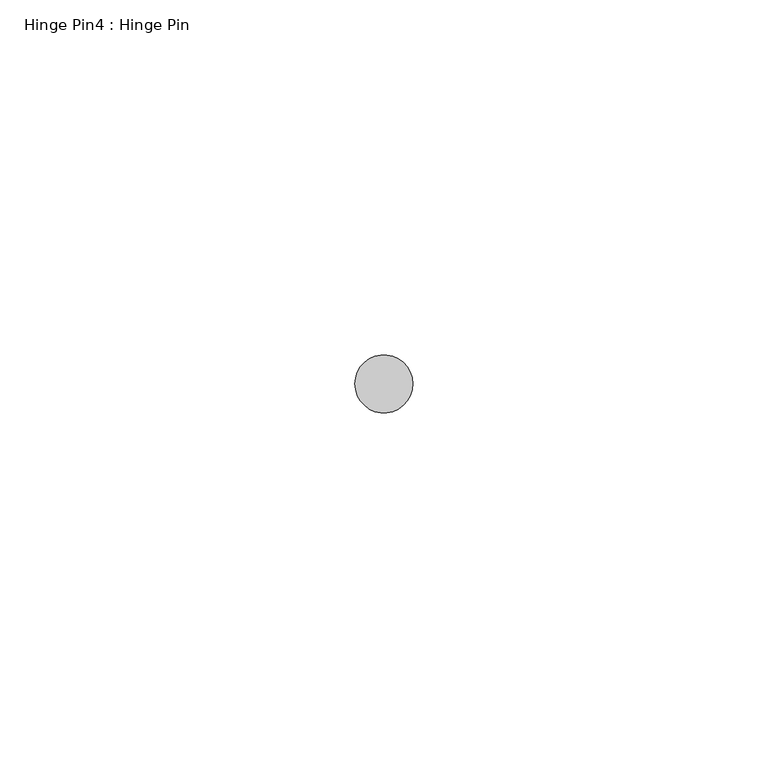
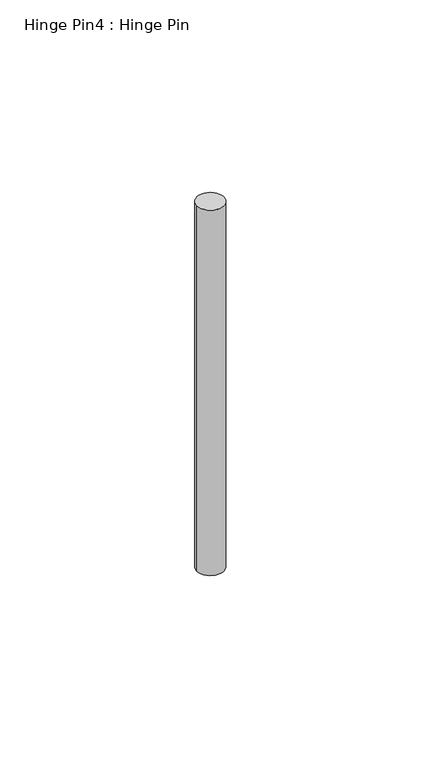
"""IFC4 building model written with IfcOpenShell, lengths in millimetres: proxy geometry, Hinge Pin4 : Hinge Pin."""

from ifc_helpers import new_model, si_unit, point, frame, frame_2d, origin, place, context, project, spatial, circle_curve, trimmed, segment, composite_curve, outline, extrude, source, transform, mapped, element, save


def hinge_pin4_hinge_pin_c21d8c14(model_context):
    return source(origin(), model_context, "Body", "SweptSolid", [
        extrude(outline(composite_curve([segment(trimmed(circle_curve(frame_2d((587319.1320739, -531776.6049841)), 4.0894), [point((587315.0426739, -531776.6049841))], [point((587323.2214739, -531776.6049841))], False, "CARTESIAN"), True, "CONTINUOUS"), segment(trimmed(circle_curve(frame_2d((587319.1320739, -531776.6049841)), 4.0894), [point((587323.2214739, -531776.6049841))], [point((587315.0426739, -531776.6049841))], False, "CARTESIAN"), True, "CONTINUOUS")], self_intersect=False)), frame((0.0, 0.0, 1128.5140625), z_axis=(0.0, 0.0, 1.0), x_axis=(1.0, 0.0, 0.0)), (0.0, 0.0, 1.0), 117.871875),
    ])


if __name__ == "__main__":
    model = new_model("IFC4")
    model_context = context("Model", 3, world=origin())
    ifc_project = project(units=[si_unit("LENGTHUNIT", "METRE", prefix="MILLI")], contexts=[model_context])
    site = spatial("IfcSite", under=ifc_project)
    building = spatial("IfcBuilding", under=site)
    placement = place(None, origin())
    hinge_pin4_hinge_pin_shape = hinge_pin4_hinge_pin_c21d8c14(model_context)
    element("IfcBuildingElementProxy", 1, Name="Hinge Pin4 : Hinge Pin", ObjectType="Hinge Pin4 : Hinge Pin", at=placement, inside=building, context=model_context, shape_type="MappedRepresentation", body=[
        mapped(hinge_pin4_hinge_pin_shape, transform((0.0, 0.0, 0.0), x_axis=(1.0, 0.0, 0.0), y_axis=(0.0, 1.0, 0.0), z_axis=(0.0, 0.0, 1.0))),
    ])
    save(model, "model.ifc")

# Revit data of these elements
# Element 1 (IfcBuildingElementProxy, "Hinge Pin4 : Hinge Pin")
#   Materials on its faces: "6\"X6\" WELD-ON STL BUTT HINGE"
# Materials
#   "6\"X6\" WELD-ON STL BUTT HINGE": class "Metal", colour RGB 189 187 185, transparency 0, Description = "Carbon steel", Cost = 0
